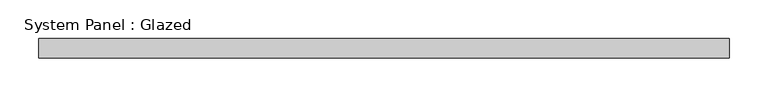
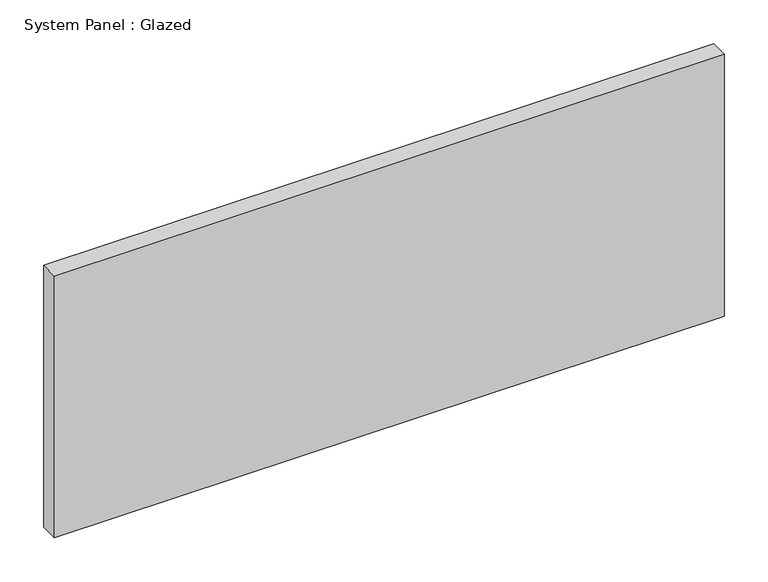
"""IFC4 building model written with IfcOpenShell, lengths in millimetres: plate geometry, System Panel : Glazed."""

import ifcopenshell
import ifcopenshell.guid

model = None  # the IFC model being written
_history = None  # IfcOwnerHistory: only IFC2X3 demands one
_inside = {}  # id of a spatial element -> (the spatial element, [elements in it])
_under = {}  # id of a project, library or spatial element -> (it, [spatial elements below it])
_declared = {}  # id of a project -> (the project, [libraries it declares])
_typed = {}  # id of a type object -> (the type object, [elements of that type])
_made_of = {}  # id of a material, layer set ... -> (it, [elements and type objects made of it])


def new_model(schema):
    """Start an empty IFC model of exactly this schema.

    Asked for "IFC4X3", IfcOpenShell would pick the latest addendum, in which some entities
    have other attributes; the version numbers below select the first issue.
    IFC2X3 requires an IfcOwnerHistory on every rooted entity: one is made here for all.
    """
    global model, _history
    if schema == "IFC4X3":
        model = ifcopenshell.file(schema_version=(4, 3, 0, 0))
    else:
        model = ifcopenshell.file(schema=schema)
    _inside.clear()
    _under.clear()
    _declared.clear()
    _typed.clear()
    _made_of.clear()
    _history = None
    if model.schema == "IFC2X3":
        org = make("IfcOrganization", Name="unknown")
        user = make(
            "IfcPersonAndOrganization",
            ThePerson=make("IfcPerson", FamilyName="unknown"),
            TheOrganization=org,
        )
        app = make(
            "IfcApplication",
            ApplicationDeveloper=org,
            Version="unknown",
            ApplicationFullName="unknown",
            ApplicationIdentifier="unknown",
        )
        _history = make(
            "IfcOwnerHistory",
            OwningUser=user,
            OwningApplication=app,
            ChangeAction="ADDED",
            CreationDate=0,
        )
    return model


def make(cls, **values):
    """One entity of the class cls with the attributes given. An attribute that is None is left unset."""
    return model.create_entity(
        cls, **{name: value for name, value in values.items() if value is not None}
    )


def rooted(cls, **values):
    """An entity with a GlobalId (a new one), such as an element, a storey or a relation."""
    return make(cls, GlobalId=ifcopenshell.guid.new(), OwnerHistory=_history, **values)


def si_unit(unit_type, name, prefix=None):
    """IfcSIUnit, for example si_unit("LENGTHUNIT", "METRE", prefix="MILLI")."""
    return make("IfcSIUnit", UnitType=unit_type, Prefix=prefix, Name=name)


def assignment(units):
    """IfcUnitAssignment: the units of a project."""
    return None if units is None else make("IfcUnitAssignment", Units=units)


def point(xyz):
    """IfcCartesianPoint."""
    return None if xyz is None else make("IfcCartesianPoint", Coordinates=xyz)


def direction(xyz):
    """IfcDirection."""
    return None if xyz is None else make("IfcDirection", DirectionRatios=xyz)


def frame(location, z_axis=None, x_axis=None):
    """IfcAxis2Placement3D, a coordinate frame: its origin and axes. An axis left out is left unset."""
    return make(
        "IfcAxis2Placement3D",
        Location=point(location),
        Axis=direction(z_axis),
        RefDirection=direction(x_axis),
    )


def origin():
    """The frame at (0, 0, 0) with its axes left unset."""
    return frame((0.0, 0.0, 0.0))


def origin_with_axes():
    """The frame at (0, 0, 0) with the z axis (0, 0, 1) and the x axis (1, 0, 0) written out."""
    return frame((0.0, 0.0, 0.0), z_axis=(0.0, 0.0, 1.0), x_axis=(1.0, 0.0, 0.0))


def place(relative_to, where):
    """IfcLocalPlacement: puts the frame where relative to a parent placement (None: the world)."""
    return make(
        "IfcLocalPlacement", PlacementRelTo=relative_to, RelativePlacement=where
    )


def context(
    kind, dimensions, precision=None, world=None, true_north=None, identifier=None
):
    """IfcGeometricRepresentationContext, for example the 3D "Model" context."""
    return make(
        "IfcGeometricRepresentationContext",
        ContextIdentifier=identifier,
        ContextType=kind,
        CoordinateSpaceDimension=dimensions,
        Precision=precision,
        WorldCoordinateSystem=world,
        TrueNorth=true_north,
    )


def project(units=None, contexts=None):
    """IfcProject with its units and contexts."""
    return rooted(
        "IfcProject",
        Name="project",
        RepresentationContexts=contexts,
        UnitsInContext=assignment(units),
    )


def spatial(cls, under=None, at=None, **own):
    """A site, building, storey or space (cls), placed at a placement, below another one or the project."""
    s = rooted(cls, ObjectPlacement=at, **own)
    if under is not None:
        _under.setdefault(under.id(), (under, []))[1].append(s)
    return s


def polyline(points):
    """IfcPolyline through the points."""
    return make("IfcPolyline", Points=[point(p) for p in points])


def outline(outer, holes=None, kind="AREA"):
    """IfcArbitraryClosedProfileDef: a profile drawn as a closed curve; with holes, ...WithVoids."""
    if holes is None:
        return make("IfcArbitraryClosedProfileDef", ProfileType=kind, OuterCurve=outer)
    return make(
        "IfcArbitraryProfileDefWithVoids",
        ProfileType=kind,
        OuterCurve=outer,
        InnerCurves=holes,
    )


def extrude(swept, where, along, depth):
    """IfcExtrudedAreaSolid: the profile swept, set in the frame where, extruded along a direction by depth."""
    return make(
        "IfcExtrudedAreaSolid",
        SweptArea=swept,
        Position=where,
        ExtrudedDirection=direction(along),
        Depth=depth,
    )


def shape(context_of_items, identifier, shape_type, items):
    """IfcShapeRepresentation: the items that make up one representation, for example the "Body"."""
    return make(
        "IfcShapeRepresentation",
        ContextOfItems=context_of_items,
        RepresentationIdentifier=identifier,
        RepresentationType=shape_type,
        Items=items,
    )


def source(mapping_origin, context_of_items, identifier, shape_type, items):
    """IfcRepresentationMap: a shape defined once, which mapped items show again and again."""
    return make(
        "IfcRepresentationMap",
        MappingOrigin=mapping_origin,
        MappedRepresentation=shape(context_of_items, identifier, shape_type, items),
    )


def transform(
    local_origin,
    x_axis=None,
    y_axis=None,
    z_axis=None,
    scale=None,
    scale2=None,
    scale3=None,
    uniform=True,
):
    """IfcCartesianTransformationOperator3D, or its non-uniform kind. x_axis, y_axis, z_axis: its Axis1, 2, 3."""
    if uniform:
        return make(
            "IfcCartesianTransformationOperator3D",
            Axis1=direction(x_axis),
            Axis2=direction(y_axis),
            LocalOrigin=point(local_origin),
            Scale=scale,
            Axis3=direction(z_axis),
        )
    return make(
        "IfcCartesianTransformationOperator3DnonUniform",
        Axis1=direction(x_axis),
        Axis2=direction(y_axis),
        LocalOrigin=point(local_origin),
        Scale=scale,
        Axis3=direction(z_axis),
        Scale2=scale2,
        Scale3=scale3,
    )


def mapped(mapping_source, mapping_target):
    """IfcMappedItem: shows the shape of a source again, moved by a transform."""
    return make(
        "IfcMappedItem", MappingSource=mapping_source, MappingTarget=mapping_target
    )


def made_of(thing, what):
    """Note that an element or type object is made of a material, layer set ...; save() writes the relation."""
    if what is not None:
        _made_of.setdefault(what.id(), (what, []))[1].append(thing)
    return thing


def element(
    cls,
    number,
    at=None,
    inside=None,
    cuts=None,
    type_object=None,
    material=None,
    context=None,
    identifier="Body",
    shape_type=None,
    held_by="IfcProductDefinitionShape",
    body=None,
    shapes=None,
    **own,
):
    """One element of the class cls, such as IfcWall. Its Tag is "e" and its number.

    at: its placement. inside: the storey or other place that contains it. cuts: it is an
    opening in that element (IfcRelVoidsElement). A single representation is given by context,
    identifier, shape_type and body (its items); several are given by shapes. held_by: the class
    of the entity that holds the representations. save() writes the other relations.
    """
    e = rooted(cls, Tag="e%d" % number, ObjectPlacement=at, **own)
    if body is not None:
        shapes = [shape(context, identifier, shape_type, body)]
    if shapes is not None:
        e.Representation = make(held_by, Representations=shapes)
    if inside is not None:
        _inside.setdefault(inside.id(), (inside, []))[1].append(e)
    if cuts is not None:
        rooted(
            "IfcRelVoidsElement", RelatingBuildingElement=cuts, RelatedOpeningElement=e
        )
    if type_object is not None:
        _typed.setdefault(type_object.id(), (type_object, []))[1].append(e)
    return made_of(e, material)


def aggregate(whole, parts):
    """IfcRelAggregates: a whole, such as a stair, and the parts it consists of."""
    return rooted("IfcRelAggregates", RelatingObject=whole, RelatedObjects=parts)


def save(model, path):
    """Write the relations noted so far, then the file.

    IfcRelAggregates (storeys below a building ...), IfcRelContainedInSpatialStructure (elements
    in a storey), IfcRelDefinesByType, IfcRelAssociatesMaterial and IfcRelDeclares: one each for
    every whole, place, type object, material and project.
    """
    for whole, parts in _under.values():
        aggregate(whole, parts)
    for where, things in _inside.values():
        rooted(
            "IfcRelContainedInSpatialStructure",
            RelatedElements=things,
            RelatingStructure=where,
        )
    for kind, things in _typed.values():
        rooted("IfcRelDefinesByType", RelatedObjects=things, RelatingType=kind)
    for what, things in _made_of.values():
        rooted("IfcRelAssociatesMaterial", RelatedObjects=things, RelatingMaterial=what)
    for by, libraries in _declared.values():
        rooted("IfcRelDeclares", RelatingContext=by, RelatedDefinitions=libraries)
    model.write(path)


def system_panel_glazed_07dea14e(model_context):
    return source(origin(), model_context, "Body", "SweptSolid", [
        extrude(outline(polyline([(443.9393939, 24.5), (-443.9393939, 24.5), (-443.9393939, 49.5), (443.9393939, 49.5), (443.9393939, 24.5)])), origin_with_axes(), (0.0, 0.0, 1.0), 366.6666667),
    ])


if __name__ == "__main__":
    model = new_model("IFC4")
    model_context = context("Model", 3, world=origin())
    ifc_project = project(units=[si_unit("LENGTHUNIT", "METRE", prefix="MILLI")], contexts=[model_context])
    site = spatial("IfcSite", under=ifc_project)
    building = spatial("IfcBuilding", under=site)
    placement = place(None, origin())
    system_panel_glazed_shape = system_panel_glazed_07dea14e(model_context)
    element("IfcPlate", 1, ObjectType="System Panel : Glazed", at=placement, inside=building, context=model_context, shape_type="MappedRepresentation", body=[
        mapped(system_panel_glazed_shape, transform((0.0, 0.0, 0.0), x_axis=(1.0, 0.0, 0.0), y_axis=(0.0, 1.0, 0.0), z_axis=(0.0, 0.0, 1.0))),
    ])
    save(model, "model.ifc")

# Revit data of these elements
# Element 1 (IfcPlate, "System Panel : Glazed")
#   Materials on its faces: "Glass"
# Materials
#   "Glass": class "Glass", colour RGB 218 227 224, transparency 0.85, Description = "Soda Lime Glass", Cost = 0
